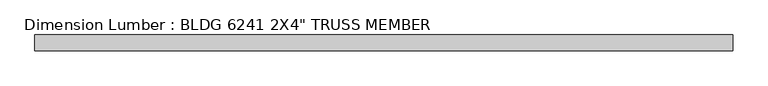
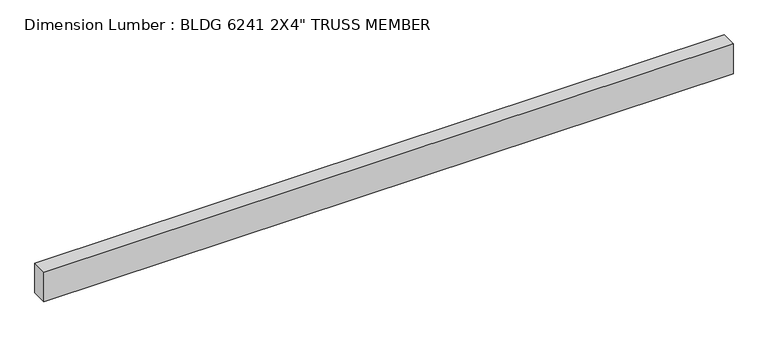
"""IFC4 building model written with IfcOpenShell, lengths in millimetres: beam geometry."""

from ifc_helpers import new_model, si_unit, frame, origin, place, context, project, spatial, polyline, outline, extrude, source, transform, mapped, element, save


def beam_50604119(model_context):
    return source(origin(), model_context, "Body", "SweptSolid", [
        extrude(outline(polyline([(1117.6, 25.4), (1117.6, -25.4), (-1117.6, -25.4), (-1117.6, 25.4), (1117.6, 25.4)])), frame((0.0, 0.0, -50.8), z_axis=(0.0, 0.0, 1.0), x_axis=(1.0, 0.0, 0.0)), (0.0, 0.0, 1.0), 101.6),
    ])


if __name__ == "__main__":
    model = new_model("IFC4")
    model_context = context("Model", 3, world=origin())
    ifc_project = project(units=[si_unit("LENGTHUNIT", "METRE", prefix="MILLI")], contexts=[model_context])
    site = spatial("IfcSite", under=ifc_project)
    building = spatial("IfcBuilding", under=site)
    placement = place(None, origin())
    beam_shape = beam_50604119(model_context)
    element("IfcBeam", 1, ObjectType="Dimension Lumber : BLDG 6241 2X4\" TRUSS MEMBER", at=placement, inside=building, context=model_context, shape_type="MappedRepresentation", body=[
        mapped(beam_shape, transform((0.0, 0.0, 0.0), x_axis=(1.0, 0.0, 0.0), y_axis=(0.0, 1.0, 0.0), z_axis=(0.0, 0.0, 1.0))),
    ])
    save(model, "model.ifc")

# Revit data of these elements
# Type "Dimension Lumber : BLDG 6241 2X4\" TRUSS MEMBER"
#   Assembly Code = "B10"
#   A = 0.273472 SF
#   Length [instance default] = 5' - 0"
#   b = 0' - 2"
#   d = 0' - 4"
#   Structural Material [instance default] = Softwood, Lumber
# Element 1 (IfcBeam, "Dimension Lumber : BLDG 6241 2X4\" TRUSS MEMBER")
#   Materials on its faces: "Softwood, Lumber"
# Materials
#   "Softwood, Lumber": class "Wood", colour RGB 223 192 134, transparency 0, Description = "Pinus Echinata", Cost = 0
